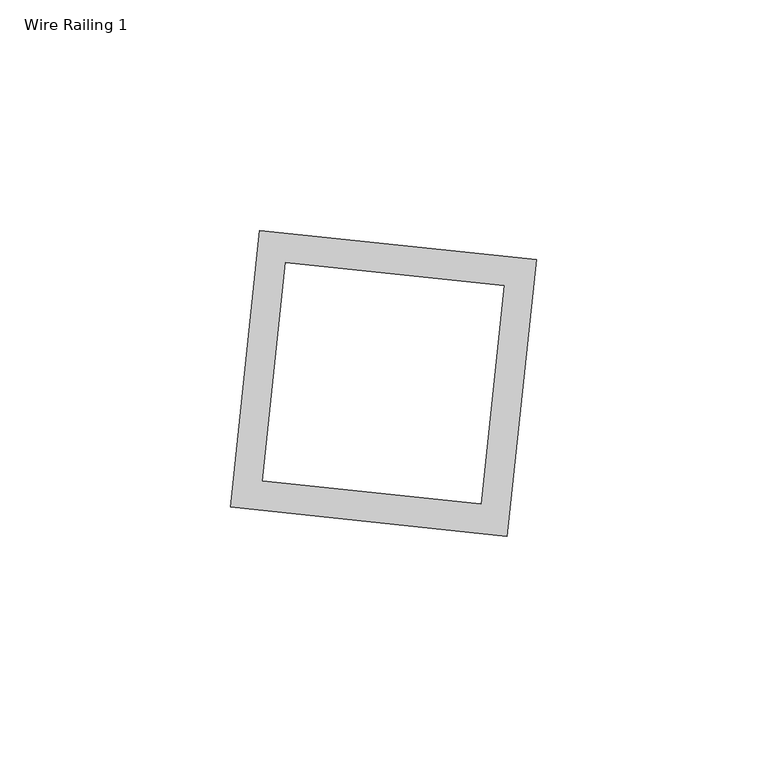
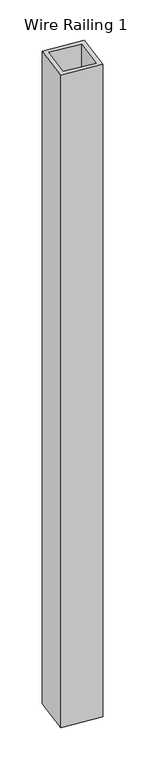
"""IFC4 building model written with IfcOpenShell, lengths in millimetres: railing geometry, Wire Railing 1."""

from ifc_helpers import new_model, si_unit, frame, origin, place, context, project, spatial, polyline, outline, extrude, source, transform, mapped, element, save


def wire_railing_1_b2c38bb6(model_context):
    return source(origin(), model_context, "Body", "SweptSolid", [
        extrude(outline(polyline([(34303.4183479, 30830.4261187), (34243.4238146, 30836.7317982), (34249.7294941, 30896.7263316), (34309.7240275, 30890.420652), (34303.4183479, 30830.4261187)]), holes=[polyline([(34297.7668896, 30837.4050885), (34302.7450577, 30884.7691937), (34255.3809524, 30889.7473618), (34250.4027844, 30842.3832565), (34297.7668896, 30837.4050885)])]), frame((0.0, 0.0, 269259.05), z_axis=(0.0, 0.0, 1.0), x_axis=(1.0, 0.0, 0.0)), (0.0, 0.0, 1.0), 1047.75),
    ])


if __name__ == "__main__":
    model = new_model("IFC4")
    model_context = context("Model", 3, world=origin())
    ifc_project = project(units=[si_unit("LENGTHUNIT", "METRE", prefix="MILLI")], contexts=[model_context])
    site = spatial("IfcSite", under=ifc_project)
    building = spatial("IfcBuilding", under=site)
    placement = place(None, origin())
    wire_railing_1_shape = wire_railing_1_b2c38bb6(model_context)
    element("IfcRailing", 1, ObjectType="Wire Railing 1", at=placement, inside=building, context=model_context, shape_type="MappedRepresentation", body=[
        mapped(wire_railing_1_shape, transform((0.0, 0.0, 0.0), x_axis=(1.0, 0.0, 0.0), y_axis=(0.0, 1.0, 0.0), z_axis=(0.0, 0.0, 1.0))),
    ])
    save(model, "model.ifc")

# Revit data of these elements
# Element 1 (IfcRailing, "Wire Railing 1")
#   Materials on its faces: "2 1/2\" X 2 1/2\" ALUM. SQUARE POST (38\" O.C. MAX)", "WIRE RAILING (3\" O.C.)", "ALUM. PLATE TOP RAIL"
# Materials
#   "2 1/2\" X 2 1/2\" ALUM. SQUARE POST (38\" O.C. MAX)": class "Metal", colour RGB 244 244 244, transparency 0, Manufacturer = "Kawneer", URL = "http://www.kawneer.com/kawneer/north_america/en/home.asp", Cost = 0
#   "WIRE RAILING (3\" O.C.)": class "Metal", colour RGB 244 244 244, transparency 0, Manufacturer = "Kawneer", URL = "http://www.kawneer.com/kawneer/north_america/en/home.asp", Cost = 0
#   "ALUM. PLATE TOP RAIL": class "Metal", colour RGB 244 244 244, transparency 0, Manufacturer = "Kawneer", URL = "http://www.kawneer.com/kawneer/north_america/en/home.asp", Cost = 0
